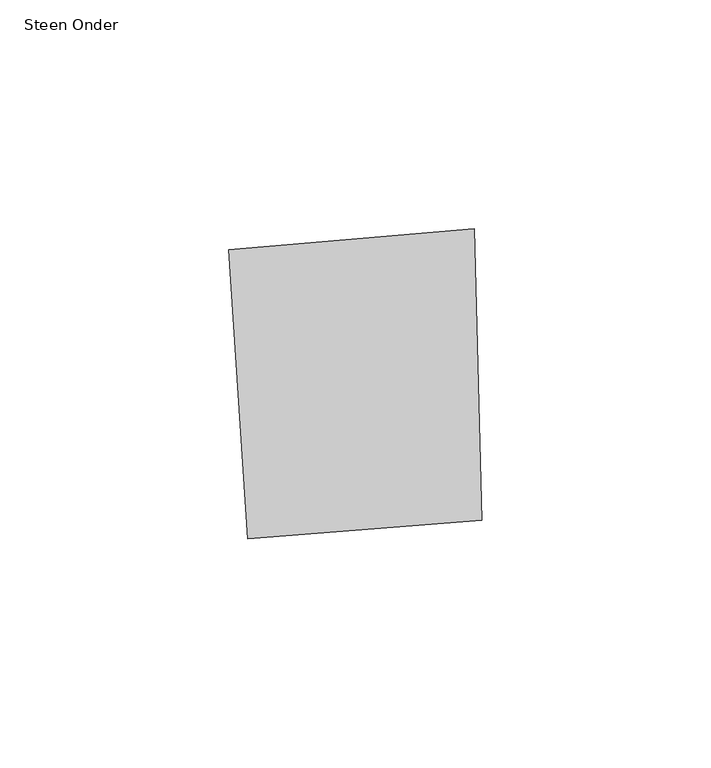
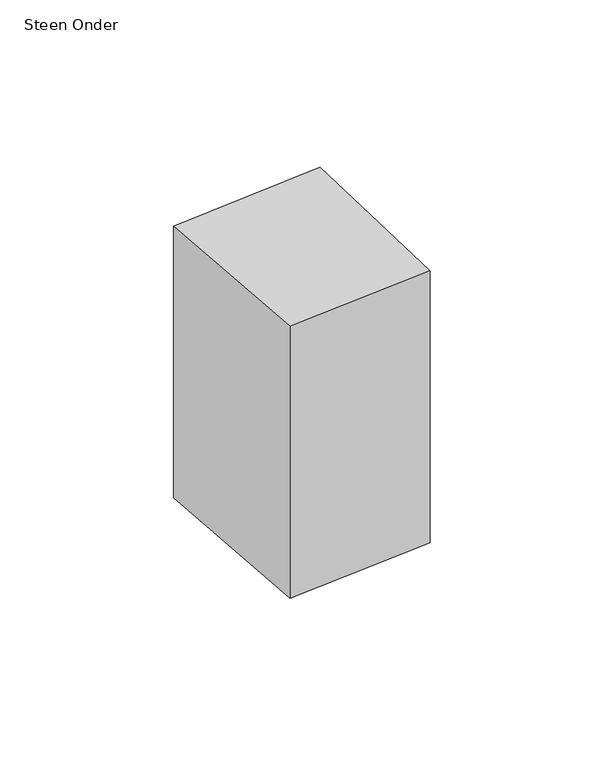
"""IFC4 building model written with IfcOpenShell, lengths in millimetres: proxy geometry, 00_GMA_steen_versie_4 : Steen Onder."""

from ifc_helpers import new_model, si_unit, origin, origin_with_axes, place, context, project, spatial, polyline, outline, extrude, source, transform, mapped, element, save


def steen_onder_03a3933b(model_context):
    return source(origin(), model_context, "Body", "SweptSolid", [
        extrude(outline(polyline([(99.8242759, 97.5496675), (101.4345345, 33.9251916), (50.3031265, 29.8489697), (46.2132648, 93.0027955), (99.8242759, 97.5496675)])), origin_with_axes(), (0.0, 0.0, 1.0), 100.0),
    ])


if __name__ == "__main__":
    model = new_model("IFC4")
    model_context = context("Model", 3, world=origin())
    ifc_project = project(units=[si_unit("LENGTHUNIT", "METRE", prefix="MILLI")], contexts=[model_context])
    site = spatial("IfcSite", under=ifc_project)
    building = spatial("IfcBuilding", under=site)
    placement = place(None, origin())
    steen_onder_shape = steen_onder_03a3933b(model_context)
    element("IfcBuildingElementProxy", 1, Name="00_GMA_steen_versie_4 : Steen Onder", ObjectType="00_GMA_steen_versie_4 : Steen Onder", at=placement, inside=building, context=model_context, shape_type="MappedRepresentation", body=[
        mapped(steen_onder_shape, transform((0.0, 0.0, 0.0), x_axis=(1.0, 0.0, 0.0), y_axis=(0.0, 1.0, 0.0), z_axis=(0.0, 0.0, 1.0))),
    ])
    save(model, "model.ifc")

# Revit data of these elements
# Type "00_GMA_steen_versie_4 : Steen Onder"
#   StootVoegHalfBoven [instance default] = 5 mm
#   StootVoegHalf [instance default] = 5 mm
#   StootVoegBreedteOnder = 10 mm
#   StootVoegBreedteBoven = 10 mm
#   Steendikte = 100 mm
#   LintVoegOnderHalf = 0 mm
#   LintVoegOnder = 0 mm
#   LintVoegBovenHalf = 5 mm
#   LintVoegBoven = 10 mm
#   materiaal = none
#   MateriaalVoeg = none
#   Default Elevation = 0
